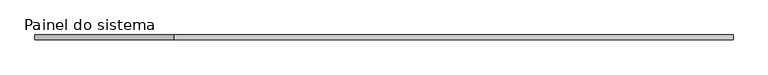
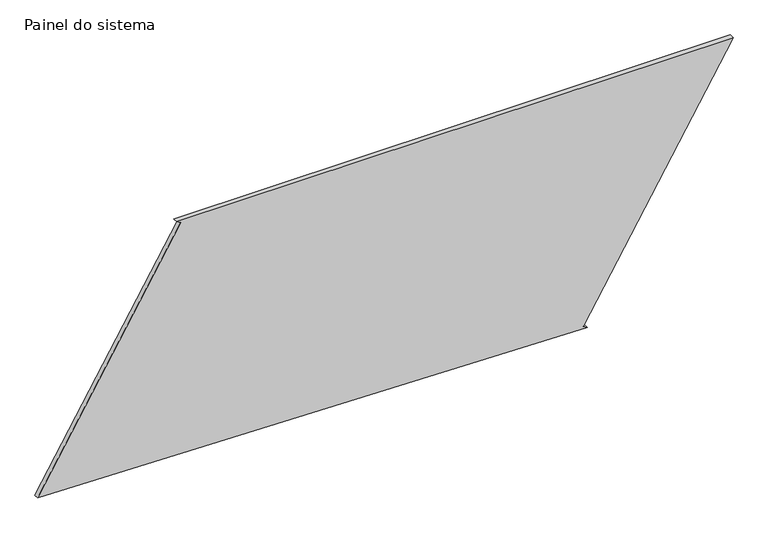
"""IFC4 building model written with IfcOpenShell, lengths in millimetres: plate geometry, Painel do sistema : Envidraçado."""

from ifc_helpers import new_model, si_unit, frame, origin, place, context, project, spatial, polyline, outline, extrude, source, transform, mapped, element, save


def painel_do_sistema_cf0d3bf1(model_context):
    return source(origin(), model_context, "Body", "SweptSolid", [
        extrude(outline(polyline([(0.0, 1073.5834282), (12.7505939, 1052.0794203), (1359.5968803, 1850.6789289), (1359.5968803, -1111.128185), (1346.8462864, -1089.6241772), (63.3196186, -1850.6789289), (0.0, 1073.5834282)])), frame((0.0, 24.5, 0.0), z_axis=(0.0, 1.0, 0.0), x_axis=(0.0, 0.0, 1.0)), (0.0, 0.0, 1.0), 25.0),
    ])


if __name__ == "__main__":
    model = new_model("IFC4")
    model_context = context("Model", 3, world=origin())
    ifc_project = project(units=[si_unit("LENGTHUNIT", "METRE", prefix="MILLI")], contexts=[model_context])
    site = spatial("IfcSite", under=ifc_project)
    building = spatial("IfcBuilding", under=site)
    placement = place(None, origin())
    painel_do_sistema_shape = painel_do_sistema_cf0d3bf1(model_context)
    element("IfcPlate", 1, ObjectType="Painel do sistema : Envidraçado", at=placement, inside=building, context=model_context, shape_type="MappedRepresentation", body=[
        mapped(painel_do_sistema_shape, transform((0.0, 0.0, 0.0), x_axis=(1.0, 0.0, 0.0), y_axis=(0.0, 1.0, 0.0), z_axis=(0.0, 0.0, 1.0))),
    ])
    save(model, "model.ifc")

# Revit data of these elements
# Type "Painel do sistema : Envidraçado"
#   Construction Type Id = "GSP4R"
#   Analytic Construction = "Vidraça única Pilkington 1/8 pol"
#   Visual Light Transmittance = 0.9
#   Solar Heat Gain Coefficient = 0.86
#   Heat Transfer Coefficient (U) = 6.7069 W/(m²·K)
# Element 1 (IfcPlate, "Painel do sistema : Envidraçado")
#   Materials on its faces: "Vidro"
# Materials
#   "Vidro": class "Vidro", colour RGB 0 128 192, transparency 0.9, Description = "Vidro de sílica", Cost = 0
